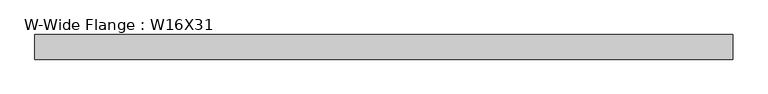
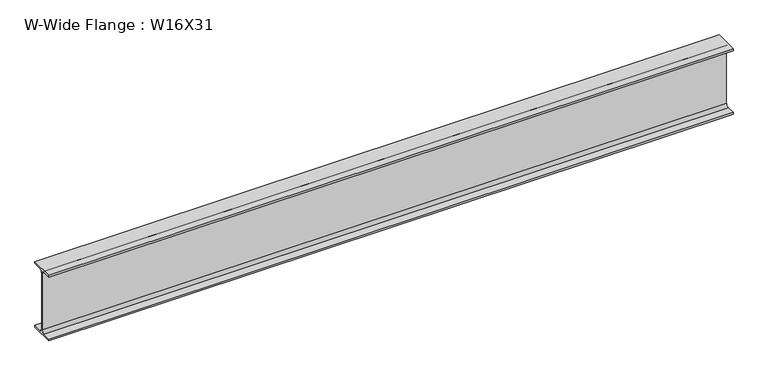
"""IFC4 building model written with IfcOpenShell, lengths in millimetres: beam geometry, W-Wide Flange : W16X31."""

from ifc_helpers import new_model, si_unit, point, frame, frame_2d, origin, place, context, project, spatial, polyline, circle_curve, trimmed, segment, composite_curve, outline, extrude, source, transform, mapped, element, save


def w_wide_flange_w16x31_3e3183ac(model_context):
    return source(origin(), model_context, "Body", "SweptSolid", [
        extrude(outline(composite_curve([segment(polyline([(70.231, -190.754), (70.231, -201.93), (-70.231, -201.93), (-70.231, -190.754), (-20.8915, -190.754)]), True, "CONTINUOUS"), segment(trimmed(circle_curve(frame_2d((-20.8915, -173.355)), 17.399), [point((-20.8915, -190.754))], [point((-3.4925, -173.355))], True, "CARTESIAN"), True, "CONTINUOUS"), segment(polyline([(-3.4925, -173.355), (-3.4925, 173.355)]), True, "CONTINUOUS"), segment(trimmed(circle_curve(frame_2d((-20.8915, 173.355)), 17.399), [point((-3.4925, 173.355))], [point((-20.8915, 190.754))], True, "CARTESIAN"), True, "CONTINUOUS"), segment(polyline([(-20.8915, 190.754), (-70.231, 190.754), (-70.231, 201.93), (70.231, 201.93), (70.231, 190.754), (20.8915, 190.754)]), True, "CONTINUOUS"), segment(trimmed(circle_curve(frame_2d((20.8915, 173.355)), 17.399), [point((20.8915, 190.754))], [point((3.4925, 173.355))], True, "CARTESIAN"), True, "CONTINUOUS"), segment(polyline([(3.4925, 173.355), (3.4925, -173.355)]), True, "CONTINUOUS"), segment(trimmed(circle_curve(frame_2d((20.8915, -173.355)), 17.399), [point((3.4925, -173.355))], [point((20.8915, -190.754))], True, "CARTESIAN"), True, "CONTINUOUS"), segment(polyline([(20.8915, -190.754), (70.231, -190.754)]), True, "CONTINUOUS")], self_intersect=False)), frame((-2052.124346, 0.0, 0.0), z_axis=(1.0, 0.0, 0.0), x_axis=(0.0, 1.0, 0.0)), (0.0, 0.0, 1.0), 3987.789692),
    ])


if __name__ == "__main__":
    model = new_model("IFC4")
    model_context = context("Model", 3, world=origin())
    ifc_project = project(units=[si_unit("LENGTHUNIT", "METRE", prefix="MILLI")], contexts=[model_context])
    site = spatial("IfcSite", under=ifc_project)
    building = spatial("IfcBuilding", under=site)
    placement = place(None, origin())
    w_wide_flange_w16x31_shape = w_wide_flange_w16x31_3e3183ac(model_context)
    element("IfcBeam", 1, ObjectType="W-Wide Flange : W16X31", at=placement, inside=building, context=model_context, shape_type="MappedRepresentation", body=[
        mapped(w_wide_flange_w16x31_shape, transform((0.0, 0.0, 0.0), x_axis=(1.0, 0.0, 0.0), y_axis=(0.0, 1.0, 0.0), z_axis=(0.0, 0.0, 1.0))),
    ])
    save(model, "model.ifc")

# Revit data of these elements
# Type "W-Wide Flange : W16X31"
#   Assembly Code = "B10"
#   W = 31
#   Start Extension Calculation [instance default] = 10' - 0"
#   Start Extension [instance default] = -0' - 0 1/2"
#   End Extension Calculation [instance default] = 10' - 0"
#   End Extension [instance default] = -0' - 0 1/2"
#   Length [instance default] = 5' - 0"
#   bf = 0' - 5.53"
#   d = 1' - 3.9"
#   k = 0' - 1 1/8"
#   k2 = 0' - 0.685"
#   tf = 0' - 0.44"
#   tw = 0' - 0.275"
#   A = 0.0634028 SF
#   Beam Material [instance default] = Metal - Steel - ASTM A992
# Element 1 (IfcBeam, "W-Wide Flange : W16X31")
#   Materials on its faces: "Metal - Steel - ASTM A992"
# Materials
#   "Metal - Steel - ASTM A992": class "Metal", colour RGB 128 0 0, transparency 0
